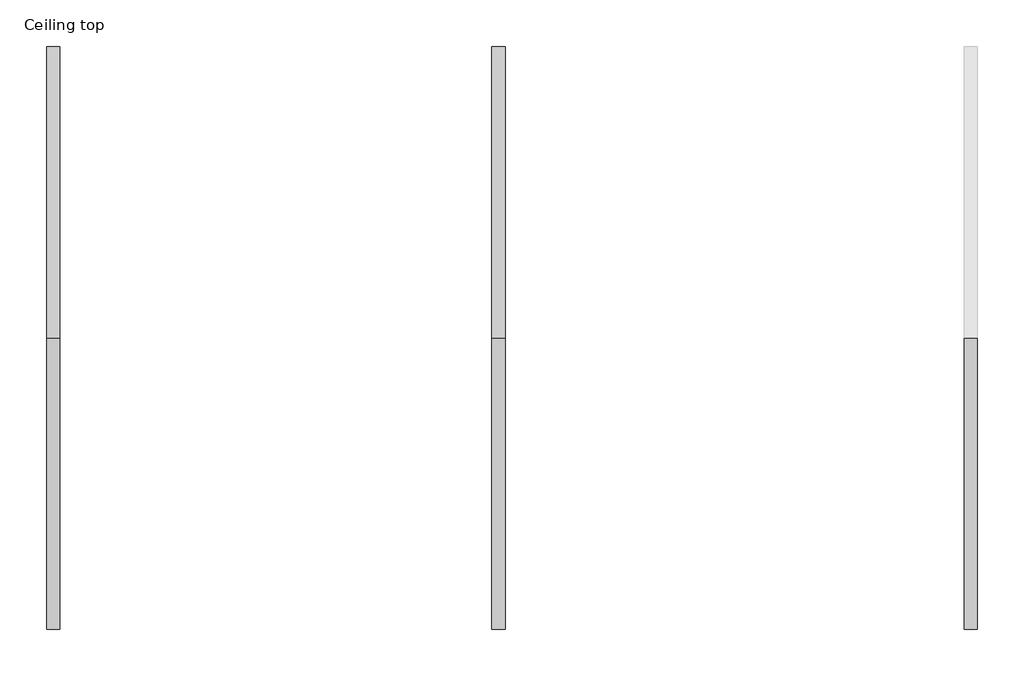
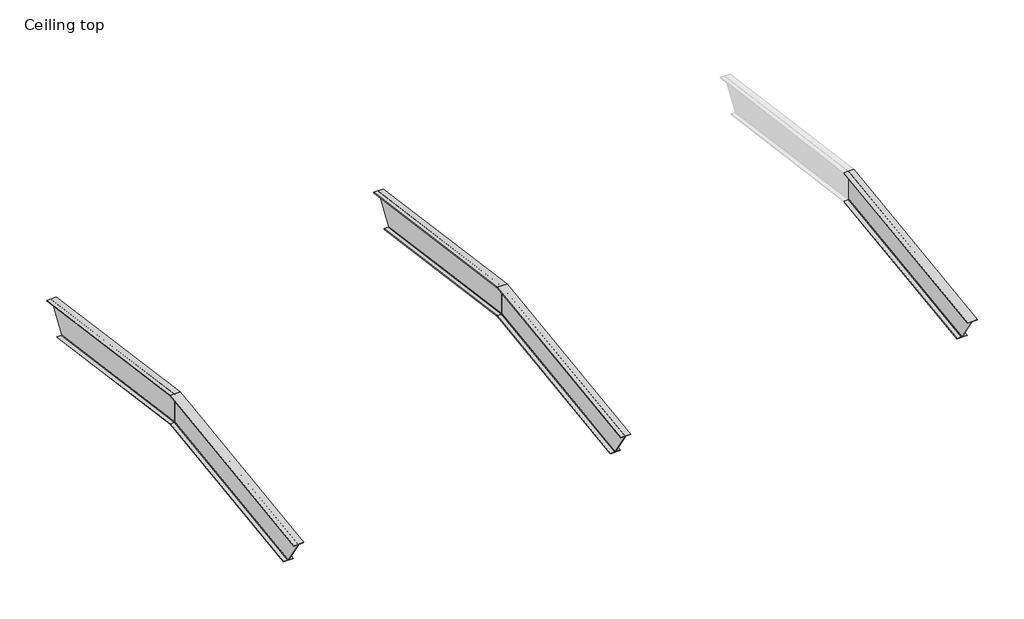
# One storey, part 1 of 2: 5 beams.
"""IFC4 building model written with IfcOpenShell, lengths in millimetres."""

from ifc_helpers import new_model, si_unit, frame, origin, place, context, project, spatial, polyline, ellipse_curve, element, save
from ifc_brep_helpers import plane_surface, revolved_surface, advanced_brep

model = new_model("IFC4")

# Units and contexts
model_context = context("Model", 3, world=origin())
ifc_project = project(units=[si_unit("LENGTHUNIT", "METRE", prefix="MILLI")], contexts=[model_context])

# Site, building, storey
site = spatial("IfcSite", under=ifc_project)
building = spatial("IfcBuilding", under=site)
storey = spatial("IfcBuildingStorey", under=building, Name="Ceiling top", Elevation=4718.05)

# Beams
placement = place(None, origin())
element("IfcBeam", 1, ObjectType="W Shapes : W 6X18.5", at=placement, inside=storey, context=model_context, shape_type="AdvancedBrep", body=[
    advanced_brep(
    [(17988.1780052, 4087.4629396, 4314.3781499), (18053.8370052, 4087.4629396, 4314.3781499), (18053.8370052, 7113.2615366, 4727.7884676), (17988.1780052, 7113.2615366, 4727.7884676), (17980.5580052, 4082.8387117, 4321.4371423), (17980.5580052, 7113.2615366, 4735.4792613), (17980.5580052, 3818.6411587, 4724.7409096), (17980.5580052, 7113.2615366, 5174.8799434), (17988.1780052, 3814.0169308, 4731.799902), (17988.1780052, 7113.2615366, 5182.5707371), (18053.8370052, 3814.0169308, 4731.799902), (18053.8370052, 7113.2615366, 5182.5707371), (18053.8370052, 3808.1595755, 4740.7412924), (18053.8370052, 7113.2615366, 5192.3124092), (17901.4370052, 3808.1595755, 4740.7412924), (17901.4370052, 7113.2615366, 5192.3124092), (17901.4370052, 3814.0169308, 4731.799902), (17901.4370052, 7113.2615366, 5182.5707371), (17967.0960052, 3814.0169308, 4731.799902), (17967.0960052, 7113.2615366, 5182.5707371), (17974.7160052, 3818.6411587, 4724.7409096), (17974.7160052, 7113.2615366, 5174.8799434), (17974.7160052, 4082.8387117, 4321.4371423), (17974.7160052, 7113.2615366, 4735.4792613), (17967.0960052, 4087.4629396, 4314.3781499), (17967.0960052, 7113.2615366, 4727.7884676), (17901.4370052, 4087.4629396, 4314.3781499), (17901.4370052, 7113.2615366, 4727.7884676), (17901.4370052, 4093.3202949, 4305.4367595), (17901.4370052, 7113.2615366, 4718.0467955), (18053.8370052, 4093.3202949, 4305.4367595), (18053.8370052, 7113.2615366, 4718.0467955)],
    [
        (0, 1),
        (1, 2),
        (2, 3),
        (3, 0),
        (4, 0, ellipse_curve(frame((17988.1780052, 4082.8387117, 4321.4371423), z_axis=(0.0, -0.8364953080573767, -0.5479740866117618), x_axis=(0.0, 0.5479740866117613, -0.8364953080573769)), 8.4387711, 7.62)),
        (3, 5, ellipse_curve(frame((17988.1780052, 7113.2615366, 4735.4792613), z_axis=(0.0, 1.0, 0.0), x_axis=(0.0, 0.0, 1.0)), 7.6907937, 7.62)),
        (5, 4),
        (6, 4),
        (5, 7),
        (7, 6),
        (8, 6, ellipse_curve(frame((17988.1780052, 3818.6411587, 4724.7409096), z_axis=(0.0, -0.8364953080573767, -0.5479740866117618), x_axis=(0.0, 0.5479740866117613, -0.8364953080573769)), 8.4387711, 7.62)),
        (7, 9, ellipse_curve(frame((17988.1780052, 7113.2615366, 5174.8799434), z_axis=(0.0, 1.0, 0.0), x_axis=(0.0, 0.0, 1.0)), 7.6907937, 7.62)),
        (9, 8),
        (10, 8),
        (9, 11),
        (11, 10),
        (12, 10),
        (11, 13),
        (13, 12),
        (14, 12),
        (13, 15),
        (15, 14),
        (16, 14),
        (15, 17),
        (17, 16),
        (18, 16),
        (17, 19),
        (19, 18),
        (20, 18, ellipse_curve(frame((17967.0960052, 3818.6411587, 4724.7409096), z_axis=(0.0, -0.8364953080573767, -0.5479740866117618), x_axis=(0.0, 0.5479740866117613, -0.8364953080573769)), 8.4387711, 7.62)),
        (19, 21, ellipse_curve(frame((17967.0960052, 7113.2615366, 5174.8799434), z_axis=(0.0, 1.0, 0.0), x_axis=(0.0, 0.0, 1.0)), 7.6907937, 7.62)),
        (21, 20),
        (22, 20),
        (21, 23),
        (23, 22),
        (24, 22, ellipse_curve(frame((17967.0960052, 4082.8387117, 4321.4371423), z_axis=(0.0, -0.8364953080573767, -0.5479740866117618), x_axis=(0.0, 0.5479740866117613, -0.8364953080573769)), 8.4387711, 7.62)),
        (23, 25, ellipse_curve(frame((17967.0960052, 7113.2615366, 4735.4792613), z_axis=(0.0, 1.0, 0.0), x_axis=(0.0, 0.0, 1.0)), 7.6907937, 7.62)),
        (25, 24),
        (26, 24),
        (25, 27),
        (27, 26),
        (28, 26),
        (27, 29),
        (29, 28),
        (30, 28),
        (29, 31),
        (31, 30),
        (1, 30),
        (31, 2),
    ],
    [
        plane_surface(frame((18053.8370052, 3870.4622337, 4284.7296694), z_axis=(0.0, -0.13537083308413533, 0.9907950027882192), x_axis=(0.0, 0.9907950027882192, 0.13537083308413533))),
        revolved_surface(polyline([(17980.5580052, 7114.293062347846, 4735.620197080616), (17980.5580052, 4079.246009561649, 4320.946276815561)]), (17988.1780052, 3869.430708, 4292.2795273), (0.0, 0.9907950027882191, 0.1353708330841353)),
        plane_surface(frame((17980.5580052, 3869.430708, 4292.2795273), z_axis=(1.0, 0.0, 0.0), x_axis=(0.0, 0.9907950027882192, 0.13537083308413533))),
        revolved_surface(polyline([(17980.5580052, 7114.293062345409, 5175.020879198452), (17980.5580052, 3815.0484565475394, 4724.2500440828635)]), (17988.1780052, 3810.4962036, 4723.6280766), (0.0, 0.9907950027882191, 0.1353708330841353)),
        plane_surface(frame((17988.1780052, 3809.4646778, 4731.1779345), z_axis=(0.0, 0.13537083308413533, -0.9907950027882192), x_axis=(0.0, 0.9907950027882192, 0.13537083308413533))),
        plane_surface(frame((18053.8370052, 3809.4646778, 4731.1779345), z_axis=(1.0, 0.0, 0.0), x_axis=(0.0, 0.9907950027882192, 0.13537083308413533))),
        plane_surface(frame((18053.8370052, 3808.1580786, 4740.7410879), z_axis=(0.0, -0.13537083308413533, 0.9907950027882192), x_axis=(0.0, 0.9907950027882192, 0.13537083308413533))),
        plane_surface(frame((17901.4370052, 3808.1580786, 4740.7410879), z_axis=(-1.0, 0.0, 0.0), x_axis=(0.0, 0.9907950027882192, 0.13537083308413533))),
        plane_surface(frame((17901.4370052, 3809.4646778, 4731.1779345), z_axis=(0.0, 0.13537083308413533, -0.9907950027882192), x_axis=(0.0, 0.9907950027882192, 0.13537083308413533))),
        revolved_surface(polyline([(17959.476005200002, 7114.293062345409, 5175.020879198452), (17959.476005200002, 3815.0484565475394, 4724.2500440828635)]), (17967.0960052, 3810.4962036, 4723.6280766), (0.0, 0.9907950027882191, 0.1353708330841353)),
        plane_surface(frame((17974.7160052, 3810.4962036, 4723.6280766), z_axis=(-1.0, 0.0, 0.0), x_axis=(0.0, 0.9907950027882192, 0.13537083308413533))),
        revolved_surface(polyline([(17959.476005200002, 7114.293062347846, 4735.620197080616), (17959.476005200002, 4079.246009561649, 4320.946276815561)]), (17967.0960052, 3869.430708, 4292.2795273), (0.0, 0.9907950027882191, 0.1353708330841353)),
        plane_surface(frame((17967.0960052, 3870.4622337, 4284.7296694), z_axis=(0.0, -0.13537083308413533, 0.9907950027882192), x_axis=(0.0, 0.9907950027882192, 0.13537083308413533))),
        plane_surface(frame((17901.4370052, 3870.4622337, 4284.7296694), z_axis=(-1.0, 0.0, 0.0), x_axis=(0.0, 0.9907950027882192, 0.13537083308413533))),
        plane_surface(frame((17901.4370052, 3871.768833, 4275.166516), z_axis=(0.0, 0.13537083308413533, -0.9907950027882192), x_axis=(0.0, 0.9907950027882192, 0.13537083308413533))),
        plane_surface(frame((18053.8370052, 3871.768833, 4275.166516), z_axis=(1.0, 0.0, 0.0), x_axis=(0.0, 0.9907950027882192, 0.13537083308413533))),
        plane_surface(frame((17977.6405771, 7113.2615366, 5192.3156137), z_axis=(0.0, 1.0, 0.0), x_axis=(0.0, 0.0, -1.0))),
        plane_surface(frame((17977.6405771, 4093.3183681, 4305.4397008), z_axis=(0.0, -0.8364953080573767, -0.5479740866117618), x_axis=(1.0, 0.0, 0.0))),
    ],
    [
        (0, [[1, 2, 3, 4]]),
        (1, [[5, -4, 6, 7]]),
        (2, [[8, -7, 9, 10]]),
        (3, [[11, -10, 12, 13]]),
        (4, [[14, -13, 15, 16]]),
        (5, [[17, -16, 18, 19]]),
        (6, [[20, -19, 21, 22]]),
        (7, [[23, -22, 24, 25]]),
        (8, [[26, -25, 27, 28]]),
        (9, [[29, -28, 30, 31]]),
        (10, [[32, -31, 33, 34]]),
        (11, [[35, -34, 36, 37]]),
        (12, [[38, -37, 39, 40]]),
        (13, [[41, -40, 42, 43]]),
        (14, [[44, -43, 45, 46]]),
        (15, [[47, -46, 48, -2]]),
        (16, [[-48, -45, -42, -39, -36, -33, -30, -27, -24, -21, -18, -15, -12, -9, -6, -3]]),
        (17, [[-1, -5, -8, -11, -14, -17, -20, -23, -26, -29, -32, -35, -38, -41, -44, -47]]),
    ],
),
])
element("IfcBeam", 2, ObjectType="W Shapes : W 6X18.5", at=placement, inside=storey, context=model_context, shape_type="AdvancedBrep", body=[
    advanced_brep(
    [(12635.1280052, 7113.2615366, 4727.7884676), (12700.7870052, 7113.2615366, 4727.7884676), (12700.7870052, 10139.0601337, 4314.3781499), (12635.1280052, 10139.0601337, 4314.3781499), (12627.5080052, 7113.2615366, 4735.4792613), (12627.5080052, 10143.6843616, 4321.4371423), (12627.5080052, 7113.2615366, 5174.8799434), (12627.5080052, 10407.8819145, 4724.7409096), (12635.1280052, 7113.2615366, 5182.5707371), (12635.1280052, 10412.5061424, 4731.799902), (12700.7870052, 7113.2615366, 5182.5707371), (12700.7870052, 10412.5061424, 4731.799902), (12700.7870052, 7113.2615366, 5192.3124092), (12700.7870052, 10418.3634977, 4740.7412924), (12548.3870052, 7113.2615366, 5192.3124092), (12548.3870052, 10418.3634977, 4740.7412924), (12548.3870052, 7113.2615366, 5182.5707371), (12548.3870052, 10412.5061424, 4731.799902), (12614.0460052, 7113.2615366, 5182.5707371), (12614.0460052, 10412.5061424, 4731.799902), (12621.6660052, 7113.2615366, 5174.8799434), (12621.6660052, 10407.8819145, 4724.7409096), (12621.6660052, 7113.2615366, 4735.4792613), (12621.6660052, 10143.6843616, 4321.4371423), (12614.0460052, 7113.2615366, 4727.7884676), (12614.0460052, 10139.0601337, 4314.3781499), (12548.3870052, 7113.2615366, 4727.7884676), (12548.3870052, 10139.0601337, 4314.3781499), (12548.3870052, 7113.2615366, 4718.0467955), (12548.3870052, 10133.2027784, 4305.4367595), (12700.7870052, 7113.2615366, 4718.0467955), (12700.7870052, 10133.2027784, 4305.4367595)],
    [
        (0, 1),
        (1, 2),
        (2, 3),
        (3, 0),
        (4, 0, ellipse_curve(frame((12635.1280052, 7113.2615366, 4735.4792613), z_axis=(0.0, -1.0, 0.0), x_axis=(0.0, 0.0, -1.0)), 7.6907937, 7.62)),
        (3, 5, ellipse_curve(frame((12635.1280052, 10143.6843616, 4321.4371423), z_axis=(0.0, 0.836495308057375, -0.5479740866117643), x_axis=(0.0, 0.547974086611764, 0.8364953080573752)), 8.4387711, 7.62)),
        (5, 4),
        (6, 4),
        (5, 7),
        (7, 6),
        (8, 6, ellipse_curve(frame((12635.1280052, 7113.2615366, 5174.8799434), z_axis=(0.0, -1.0, 0.0), x_axis=(0.0, 0.0, -1.0)), 7.6907937, 7.62)),
        (7, 9, ellipse_curve(frame((12635.1280052, 10407.8819145, 4724.7409096), z_axis=(0.0, 0.836495308057375, -0.5479740866117643), x_axis=(0.0, 0.547974086611764, 0.8364953080573752)), 8.4387711, 7.62)),
        (9, 8),
        (10, 8),
        (9, 11),
        (11, 10),
        (12, 10),
        (11, 13),
        (13, 12),
        (14, 12),
        (13, 15),
        (15, 14),
        (16, 14),
        (15, 17),
        (17, 16),
        (18, 16),
        (17, 19),
        (19, 18),
        (20, 18, ellipse_curve(frame((12614.0460052, 7113.2615366, 5174.8799434), z_axis=(0.0, -1.0, 0.0), x_axis=(0.0, 0.0, -1.0)), 7.6907937, 7.62)),
        (19, 21, ellipse_curve(frame((12614.0460052, 10407.8819145, 4724.7409096), z_axis=(0.0, 0.836495308057375, -0.5479740866117643), x_axis=(0.0, 0.547974086611764, 0.8364953080573752)), 8.4387711, 7.62)),
        (21, 20),
        (22, 20),
        (21, 23),
        (23, 22),
        (24, 22, ellipse_curve(frame((12614.0460052, 7113.2615366, 4735.4792613), z_axis=(0.0, -1.0, 0.0), x_axis=(0.0, 0.0, -1.0)), 7.6907937, 7.62)),
        (23, 25, ellipse_curve(frame((12614.0460052, 10143.6843616, 4321.4371423), z_axis=(0.0, 0.836495308057375, -0.5479740866117643), x_axis=(0.0, 0.547974086611764, 0.8364953080573752)), 8.4387711, 7.62)),
        (25, 24),
        (26, 24),
        (25, 27),
        (27, 26),
        (28, 26),
        (27, 29),
        (29, 28),
        (30, 28),
        (29, 31),
        (31, 30),
        (1, 30),
        (31, 2),
    ],
    [
        plane_surface(frame((12700.7870052, 7050.9569516, 4736.3010494), z_axis=(0.0, 0.1353708330841357, 0.9907950027882191), x_axis=(0.0, 0.9907950027882191, -0.1353708330841357))),
        revolved_surface(polyline([(12627.5080052, 10147.277063747912, 4320.946276885532), (12627.5080052, 7112.230010863546, 4735.620197164001)]), (12635.1280052, 7051.9884774, 4743.8509074), (0.0, 0.9907950027882191, -0.1353708330841357)),
        plane_surface(frame((12627.5080052, 7051.9884774, 4743.8509074), z_axis=(1.0, 0.0, 0.0), x_axis=(0.0, 0.9907950027882191, -0.1353708330841357))),
        revolved_surface(polyline([(12627.5080052, 10411.474616650441, 4724.25004406808), (12627.5080052, 7112.230010852571, 5175.020879183669)]), (12635.1280052, 7110.9229818, 5175.1994566), (0.0, 0.9907950027882191, -0.1353708330841357)),
        plane_surface(frame((12635.1280052, 7111.9545075, 5182.7493145), z_axis=(0.0, -0.1353708330841357, -0.9907950027882191), x_axis=(0.0, 0.9907950027882191, -0.1353708330841357))),
        plane_surface(frame((12700.7870052, 7111.9545075, 5182.7493145), z_axis=(1.0, 0.0, 0.0), x_axis=(0.0, 0.9907950027882191, -0.1353708330841357))),
        plane_surface(frame((12700.7870052, 7113.2611068, 5192.3124679), z_axis=(0.0, 0.1353708330841357, 0.9907950027882191), x_axis=(0.0, 0.9907950027882191, -0.1353708330841357))),
        plane_surface(frame((12548.3870052, 7113.2611068, 5192.3124679), z_axis=(-1.0, 0.0, 0.0), x_axis=(0.0, 0.9907950027882191, -0.1353708330841357))),
        plane_surface(frame((12548.3870052, 7111.9545075, 5182.7493145), z_axis=(0.0, -0.1353708330841357, -0.9907950027882191), x_axis=(0.0, 0.9907950027882191, -0.1353708330841357))),
        revolved_surface(polyline([(12606.426005199999, 10411.474616650441, 4724.25004406808), (12606.426005199999, 7112.230010852571, 5175.020879183669)]), (12614.0460052, 7110.9229818, 5175.1994566), (0.0, 0.9907950027882191, -0.1353708330841357)),
        plane_surface(frame((12621.6660052, 7110.9229818, 5175.1994566), z_axis=(-1.0, 0.0, 0.0), x_axis=(0.0, 0.9907950027882191, -0.1353708330841357))),
        revolved_surface(polyline([(12606.426005199999, 10147.277063747912, 4320.946276885532), (12606.426005199999, 7112.230010863546, 4735.620197164001)]), (12614.0460052, 7051.9884774, 4743.8509074), (0.0, 0.9907950027882191, -0.1353708330841357)),
        plane_surface(frame((12614.0460052, 7050.9569516, 4736.3010494), z_axis=(0.0, 0.1353708330841357, 0.9907950027882191), x_axis=(0.0, 0.9907950027882191, -0.1353708330841357))),
        plane_surface(frame((12548.3870052, 7050.9569516, 4736.3010494), z_axis=(-1.0, 0.0, 0.0), x_axis=(0.0, 0.9907950027882191, -0.1353708330841357))),
        plane_surface(frame((12548.3870052, 7049.6503524, 4726.7378961), z_axis=(0.0, -0.1353708330841357, -0.9907950027882191), x_axis=(0.0, 0.9907950027882191, -0.1353708330841357))),
        plane_surface(frame((12700.7870052, 7049.6503524, 4726.7378961), z_axis=(1.0, 0.0, 0.0), x_axis=(0.0, 0.9907950027882191, -0.1353708330841357))),
        plane_surface(frame((12624.5905771, 7113.2615366, 5192.3156137), z_axis=(0.0, -1.0, 0.0), x_axis=(0.0, 0.0, 1.0))),
        plane_surface(frame((12624.5905771, 10418.3654245, 4740.7442336), z_axis=(0.0, 0.836495308057375, -0.5479740866117643), x_axis=(1.0, 0.0, 0.0))),
    ],
    [
        (0, [[1, 2, 3, 4]]),
        (1, [[5, -4, 6, 7]]),
        (2, [[8, -7, 9, 10]]),
        (3, [[11, -10, 12, 13]]),
        (4, [[14, -13, 15, 16]]),
        (5, [[17, -16, 18, 19]]),
        (6, [[20, -19, 21, 22]]),
        (7, [[23, -22, 24, 25]]),
        (8, [[26, -25, 27, 28]]),
        (9, [[29, -28, 30, 31]]),
        (10, [[32, -31, 33, 34]]),
        (11, [[35, -34, 36, 37]]),
        (12, [[38, -37, 39, 40]]),
        (13, [[41, -40, 42, 43]]),
        (14, [[44, -43, 45, 46]]),
        (15, [[47, -46, 48, -2]]),
        (16, [[-1, -5, -8, -11, -14, -17, -20, -23, -26, -29, -32, -35, -38, -41, -44, -47]]),
        (17, [[-48, -45, -42, -39, -36, -33, -30, -27, -24, -21, -18, -15, -12, -9, -6, -3]]),
    ],
),
])
element("IfcBeam", 3, ObjectType="W Shapes : W 6X18.5", at=placement, inside=storey, context=model_context, shape_type="AdvancedBrep", body=[
    advanced_brep(
    [(12635.1280052, 4087.4629396, 4314.3781499), (12700.7870052, 4087.4629396, 4314.3781499), (12700.7870052, 7113.2615366, 4727.7884676), (12635.1280052, 7113.2615366, 4727.7884676), (12627.5080052, 4082.8387117, 4321.4371423), (12627.5080052, 7113.2615366, 4735.4792613), (12627.5080052, 3818.6411587, 4724.7409096), (12627.5080052, 7113.2615366, 5174.8799434), (12635.1280052, 3814.0169308, 4731.799902), (12635.1280052, 7113.2615366, 5182.5707371), (12700.7870052, 3814.0169308, 4731.799902), (12700.7870052, 7113.2615366, 5182.5707371), (12700.7870052, 3808.1595755, 4740.7412924), (12700.7870052, 7113.2615366, 5192.3124092), (12548.3870052, 3808.1595755, 4740.7412924), (12548.3870052, 7113.2615366, 5192.3124092), (12548.3870052, 3814.0169308, 4731.799902), (12548.3870052, 7113.2615366, 5182.5707371), (12614.0460052, 3814.0169308, 4731.799902), (12614.0460052, 7113.2615366, 5182.5707371), (12621.6660052, 3818.6411587, 4724.7409096), (12621.6660052, 7113.2615366, 5174.8799434), (12621.6660052, 4082.8387117, 4321.4371423), (12621.6660052, 7113.2615366, 4735.4792613), (12614.0460052, 4087.4629396, 4314.3781499), (12614.0460052, 7113.2615366, 4727.7884676), (12548.3870052, 4087.4629396, 4314.3781499), (12548.3870052, 7113.2615366, 4727.7884676), (12548.3870052, 4093.3202949, 4305.4367595), (12548.3870052, 7113.2615366, 4718.0467955), (12700.7870052, 4093.3202949, 4305.4367595), (12700.7870052, 7113.2615366, 4718.0467955)],
    [
        (0, 1),
        (1, 2),
        (2, 3),
        (3, 0),
        (4, 0, ellipse_curve(frame((12635.1280052, 4082.8387117, 4321.4371423), z_axis=(0.0, -0.8364953080573767, -0.5479740866117618), x_axis=(0.0, 0.5479740866117613, -0.8364953080573769)), 8.4387711, 7.62)),
        (3, 5, ellipse_curve(frame((12635.1280052, 7113.2615366, 4735.4792613), z_axis=(0.0, 1.0, 0.0), x_axis=(0.0, 0.0, 1.0)), 7.6907937, 7.62)),
        (5, 4),
        (6, 4),
        (5, 7),
        (7, 6),
        (8, 6, ellipse_curve(frame((12635.1280052, 3818.6411587, 4724.7409096), z_axis=(0.0, -0.8364953080573767, -0.5479740866117618), x_axis=(0.0, 0.5479740866117613, -0.8364953080573769)), 8.4387711, 7.62)),
        (7, 9, ellipse_curve(frame((12635.1280052, 7113.2615366, 5174.8799434), z_axis=(0.0, 1.0, 0.0), x_axis=(0.0, 0.0, 1.0)), 7.6907937, 7.62)),
        (9, 8),
        (10, 8),
        (9, 11),
        (11, 10),
        (12, 10),
        (11, 13),
        (13, 12),
        (14, 12),
        (13, 15),
        (15, 14),
        (16, 14),
        (15, 17),
        (17, 16),
        (18, 16),
        (17, 19),
        (19, 18),
        (20, 18, ellipse_curve(frame((12614.0460052, 3818.6411587, 4724.7409096), z_axis=(0.0, -0.8364953080573767, -0.5479740866117618), x_axis=(0.0, 0.5479740866117613, -0.8364953080573769)), 8.4387711, 7.62)),
        (19, 21, ellipse_curve(frame((12614.0460052, 7113.2615366, 5174.8799434), z_axis=(0.0, 1.0, 0.0), x_axis=(0.0, 0.0, 1.0)), 7.6907937, 7.62)),
        (21, 20),
        (22, 20),
        (21, 23),
        (23, 22),
        (24, 22, ellipse_curve(frame((12614.0460052, 4082.8387117, 4321.4371423), z_axis=(0.0, -0.8364953080573767, -0.5479740866117618), x_axis=(0.0, 0.5479740866117613, -0.8364953080573769)), 8.4387711, 7.62)),
        (23, 25, ellipse_curve(frame((12614.0460052, 7113.2615366, 4735.4792613), z_axis=(0.0, 1.0, 0.0), x_axis=(0.0, 0.0, 1.0)), 7.6907937, 7.62)),
        (25, 24),
        (26, 24),
        (25, 27),
        (27, 26),
        (28, 26),
        (27, 29),
        (29, 28),
        (30, 28),
        (29, 31),
        (31, 30),
        (1, 30),
        (31, 2),
    ],
    [
        plane_surface(frame((12700.7870052, 3870.4622337, 4284.7296694), z_axis=(0.0, -0.13537083308413533, 0.9907950027882192), x_axis=(0.0, 0.9907950027882192, 0.13537083308413533))),
        revolved_surface(polyline([(12627.5080052, 7114.293062347846, 4735.620197080616), (12627.5080052, 4079.246009561649, 4320.946276815561)]), (12635.1280052, 3869.430708, 4292.2795273), (0.0, 0.9907950027882191, 0.1353708330841353)),
        plane_surface(frame((12627.5080052, 3869.430708, 4292.2795273), z_axis=(1.0, 0.0, 0.0), x_axis=(0.0, 0.9907950027882192, 0.13537083308413533))),
        revolved_surface(polyline([(12627.5080052, 7114.293062345409, 5175.020879198452), (12627.5080052, 3815.0484565475394, 4724.2500440828635)]), (12635.1280052, 3810.4962036, 4723.6280766), (0.0, 0.9907950027882191, 0.1353708330841353)),
        plane_surface(frame((12635.1280052, 3809.4646778, 4731.1779345), z_axis=(0.0, 0.13537083308413533, -0.9907950027882192), x_axis=(0.0, 0.9907950027882192, 0.13537083308413533))),
        plane_surface(frame((12700.7870052, 3809.4646778, 4731.1779345), z_axis=(1.0, 0.0, 0.0), x_axis=(0.0, 0.9907950027882192, 0.13537083308413533))),
        plane_surface(frame((12700.7870052, 3808.1580786, 4740.7410879), z_axis=(0.0, -0.13537083308413533, 0.9907950027882192), x_axis=(0.0, 0.9907950027882192, 0.13537083308413533))),
        plane_surface(frame((12548.3870052, 3808.1580786, 4740.7410879), z_axis=(-1.0, 0.0, 0.0), x_axis=(0.0, 0.9907950027882192, 0.13537083308413533))),
        plane_surface(frame((12548.3870052, 3809.4646778, 4731.1779345), z_axis=(0.0, 0.13537083308413533, -0.9907950027882192), x_axis=(0.0, 0.9907950027882192, 0.13537083308413533))),
        revolved_surface(polyline([(12606.426005199999, 7114.293062345409, 5175.020879198452), (12606.426005199999, 3815.0484565475394, 4724.2500440828635)]), (12614.0460052, 3810.4962036, 4723.6280766), (0.0, 0.9907950027882191, 0.1353708330841353)),
        plane_surface(frame((12621.6660052, 3810.4962036, 4723.6280766), z_axis=(-1.0, 0.0, 0.0), x_axis=(0.0, 0.9907950027882192, 0.13537083308413533))),
        revolved_surface(polyline([(12606.426005199999, 7114.293062347846, 4735.620197080616), (12606.426005199999, 4079.246009561649, 4320.946276815561)]), (12614.0460052, 3869.430708, 4292.2795273), (0.0, 0.9907950027882191, 0.1353708330841353)),
        plane_surface(frame((12614.0460052, 3870.4622337, 4284.7296694), z_axis=(0.0, -0.13537083308413533, 0.9907950027882192), x_axis=(0.0, 0.9907950027882192, 0.13537083308413533))),
        plane_surface(frame((12548.3870052, 3870.4622337, 4284.7296694), z_axis=(-1.0, 0.0, 0.0), x_axis=(0.0, 0.9907950027882192, 0.13537083308413533))),
        plane_surface(frame((12548.3870052, 3871.768833, 4275.166516), z_axis=(0.0, 0.13537083308413533, -0.9907950027882192), x_axis=(0.0, 0.9907950027882192, 0.13537083308413533))),
        plane_surface(frame((12700.7870052, 3871.768833, 4275.166516), z_axis=(1.0, 0.0, 0.0), x_axis=(0.0, 0.9907950027882192, 0.13537083308413533))),
        plane_surface(frame((12624.5905771, 7113.2615366, 5192.3156137), z_axis=(0.0, 1.0, 0.0), x_axis=(0.0, 0.0, -1.0))),
        plane_surface(frame((12624.5905771, 4093.3183681, 4305.4397008), z_axis=(0.0, -0.8364953080573767, -0.5479740866117618), x_axis=(1.0, 0.0, 0.0))),
    ],
    [
        (0, [[1, 2, 3, 4]]),
        (1, [[5, -4, 6, 7]]),
        (2, [[8, -7, 9, 10]]),
        (3, [[11, -10, 12, 13]]),
        (4, [[14, -13, 15, 16]]),
        (5, [[17, -16, 18, 19]]),
        (6, [[20, -19, 21, 22]]),
        (7, [[23, -22, 24, 25]]),
        (8, [[26, -25, 27, 28]]),
        (9, [[29, -28, 30, 31]]),
        (10, [[32, -31, 33, 34]]),
        (11, [[35, -34, 36, 37]]),
        (12, [[38, -37, 39, 40]]),
        (13, [[41, -40, 42, 43]]),
        (14, [[44, -43, 45, 46]]),
        (15, [[47, -46, 48, -2]]),
        (16, [[-48, -45, -42, -39, -36, -33, -30, -27, -24, -21, -18, -15, -12, -9, -6, -3]]),
        (17, [[-1, -5, -8, -11, -14, -17, -20, -23, -26, -29, -32, -35, -38, -41, -44, -47]]),
    ],
),
])
element("IfcBeam", 4, ObjectType="W Shapes : W 6X18.5", at=placement, inside=storey, context=model_context, shape_type="AdvancedBrep", body=[
    advanced_brep(
    [(7586.8780052, 7113.2615366, 4727.7884676), (7652.5370052, 7113.2615366, 4727.7884676), (7652.5370052, 10139.0601337, 4314.3781499), (7586.8780052, 10139.0601337, 4314.3781499), (7579.2580052, 7113.2615366, 4735.4792613), (7579.2580052, 10143.6843616, 4321.4371423), (7579.2580052, 7113.2615366, 5174.8799434), (7579.2580052, 10407.8819145, 4724.7409096), (7586.8780052, 7113.2615366, 5182.5707371), (7586.8780052, 10412.5061424, 4731.799902), (7652.5370052, 7113.2615366, 5182.5707371), (7652.5370052, 10412.5061424, 4731.799902), (7652.5370052, 7113.2615366, 5192.3124092), (7652.5370052, 10418.3634977, 4740.7412924), (7500.1370052, 7113.2615366, 5192.3124092), (7500.1370052, 10418.3634977, 4740.7412924), (7500.1370052, 7113.2615366, 5182.5707371), (7500.1370052, 10412.5061424, 4731.799902), (7565.7960052, 7113.2615366, 5182.5707371), (7565.7960052, 10412.5061424, 4731.799902), (7573.4160052, 7113.2615366, 5174.8799434), (7573.4160052, 10407.8819145, 4724.7409096), (7573.4160052, 7113.2615366, 4735.4792613), (7573.4160052, 10143.6843616, 4321.4371423), (7565.7960052, 7113.2615366, 4727.7884676), (7565.7960052, 10139.0601337, 4314.3781499), (7500.1370052, 7113.2615366, 4727.7884676), (7500.1370052, 10139.0601337, 4314.3781499), (7500.1370052, 7113.2615366, 4718.0467955), (7500.1370052, 10133.2027784, 4305.4367595), (7652.5370052, 7113.2615366, 4718.0467955), (7652.5370052, 10133.2027784, 4305.4367595)],
    [
        (0, 1),
        (1, 2),
        (2, 3),
        (3, 0),
        (4, 0, ellipse_curve(frame((7586.8780052, 7113.2615366, 4735.4792613), z_axis=(0.0, -1.0, 0.0), x_axis=(0.0, 0.0, -1.0)), 7.6907937, 7.62)),
        (3, 5, ellipse_curve(frame((7586.8780052, 10143.6843616, 4321.4371423), z_axis=(0.0, 0.836495308057375, -0.5479740866117643), x_axis=(0.0, 0.547974086611764, 0.8364953080573752)), 8.4387711, 7.62)),
        (5, 4),
        (6, 4),
        (5, 7),
        (7, 6),
        (8, 6, ellipse_curve(frame((7586.8780052, 7113.2615366, 5174.8799434), z_axis=(0.0, -1.0, 0.0), x_axis=(0.0, 0.0, -1.0)), 7.6907937, 7.62)),
        (7, 9, ellipse_curve(frame((7586.8780052, 10407.8819145, 4724.7409096), z_axis=(0.0, 0.836495308057375, -0.5479740866117643), x_axis=(0.0, 0.547974086611764, 0.8364953080573752)), 8.4387711, 7.62)),
        (9, 8),
        (10, 8),
        (9, 11),
        (11, 10),
        (12, 10),
        (11, 13),
        (13, 12),
        (14, 12),
        (13, 15),
        (15, 14),
        (16, 14),
        (15, 17),
        (17, 16),
        (18, 16),
        (17, 19),
        (19, 18),
        (20, 18, ellipse_curve(frame((7565.7960052, 7113.2615366, 5174.8799434), z_axis=(0.0, -1.0, 0.0), x_axis=(0.0, 0.0, -1.0)), 7.6907937, 7.62)),
        (19, 21, ellipse_curve(frame((7565.7960052, 10407.8819145, 4724.7409096), z_axis=(0.0, 0.836495308057375, -0.5479740866117643), x_axis=(0.0, 0.547974086611764, 0.8364953080573752)), 8.4387711, 7.62)),
        (21, 20),
        (22, 20),
        (21, 23),
        (23, 22),
        (24, 22, ellipse_curve(frame((7565.7960052, 7113.2615366, 4735.4792613), z_axis=(0.0, -1.0, 0.0), x_axis=(0.0, 0.0, -1.0)), 7.6907937, 7.62)),
        (23, 25, ellipse_curve(frame((7565.7960052, 10143.6843616, 4321.4371423), z_axis=(0.0, 0.836495308057375, -0.5479740866117643), x_axis=(0.0, 0.547974086611764, 0.8364953080573752)), 8.4387711, 7.62)),
        (25, 24),
        (26, 24),
        (25, 27),
        (27, 26),
        (28, 26),
        (27, 29),
        (29, 28),
        (30, 28),
        (29, 31),
        (31, 30),
        (1, 30),
        (31, 2),
    ],
    [
        plane_surface(frame((7652.5370052, 7050.9569516, 4736.3010494), z_axis=(0.0, 0.1353708330841357, 0.9907950027882191), x_axis=(0.0, 0.9907950027882191, -0.1353708330841357))),
        revolved_surface(polyline([(7579.2580052, 10147.277063747912, 4320.946276885532), (7579.2580052, 7112.230010863546, 4735.620197164001)]), (7586.8780052, 7051.9884774, 4743.8509074), (0.0, 0.9907950027882191, -0.1353708330841357)),
        plane_surface(frame((7579.2580052, 7051.9884774, 4743.8509074), z_axis=(1.0, 0.0, 0.0), x_axis=(0.0, 0.9907950027882191, -0.1353708330841357))),
        revolved_surface(polyline([(7579.2580052, 10411.474616650441, 4724.25004406808), (7579.2580052, 7112.230010852571, 5175.020879183669)]), (7586.8780052, 7110.9229818, 5175.1994566), (0.0, 0.9907950027882191, -0.1353708330841357)),
        plane_surface(frame((7586.8780052, 7111.9545075, 5182.7493145), z_axis=(0.0, -0.1353708330841357, -0.9907950027882191), x_axis=(0.0, 0.9907950027882191, -0.1353708330841357))),
        plane_surface(frame((7652.5370052, 7111.9545075, 5182.7493145), z_axis=(1.0, 0.0, 0.0), x_axis=(0.0, 0.9907950027882191, -0.1353708330841357))),
        plane_surface(frame((7652.5370052, 7113.2611068, 5192.3124679), z_axis=(0.0, 0.1353708330841357, 0.9907950027882191), x_axis=(0.0, 0.9907950027882191, -0.1353708330841357))),
        plane_surface(frame((7500.1370052, 7113.2611068, 5192.3124679), z_axis=(-1.0, 0.0, 0.0), x_axis=(0.0, 0.9907950027882191, -0.1353708330841357))),
        plane_surface(frame((7500.1370052, 7111.9545075, 5182.7493145), z_axis=(0.0, -0.1353708330841357, -0.9907950027882191), x_axis=(0.0, 0.9907950027882191, -0.1353708330841357))),
        revolved_surface(polyline([(7558.1760052, 10411.474616650441, 4724.25004406808), (7558.1760052, 7112.230010852571, 5175.020879183669)]), (7565.7960052, 7110.9229818, 5175.1994566), (0.0, 0.9907950027882191, -0.1353708330841357)),
        plane_surface(frame((7573.4160052, 7110.9229818, 5175.1994566), z_axis=(-1.0, 0.0, 0.0), x_axis=(0.0, 0.9907950027882191, -0.1353708330841357))),
        revolved_surface(polyline([(7558.1760052, 10147.277063747912, 4320.946276885532), (7558.1760052, 7112.230010863546, 4735.620197164001)]), (7565.7960052, 7051.9884774, 4743.8509074), (0.0, 0.9907950027882191, -0.1353708330841357)),
        plane_surface(frame((7565.7960052, 7050.9569516, 4736.3010494), z_axis=(0.0, 0.1353708330841357, 0.9907950027882191), x_axis=(0.0, 0.9907950027882191, -0.1353708330841357))),
        plane_surface(frame((7500.1370052, 7050.9569516, 4736.3010494), z_axis=(-1.0, 0.0, 0.0), x_axis=(0.0, 0.9907950027882191, -0.1353708330841357))),
        plane_surface(frame((7500.1370052, 7049.6503524, 4726.7378961), z_axis=(0.0, -0.1353708330841357, -0.9907950027882191), x_axis=(0.0, 0.9907950027882191, -0.1353708330841357))),
        plane_surface(frame((7652.5370052, 7049.6503524, 4726.7378961), z_axis=(1.0, 0.0, 0.0), x_axis=(0.0, 0.9907950027882191, -0.1353708330841357))),
        plane_surface(frame((7576.3405771, 7113.2615366, 5192.3156137), z_axis=(0.0, -1.0, 0.0), x_axis=(0.0, 0.0, 1.0))),
        plane_surface(frame((7576.3405771, 10418.3654245, 4740.7442336), z_axis=(0.0, 0.836495308057375, -0.5479740866117643), x_axis=(1.0, 0.0, 0.0))),
    ],
    [
        (0, [[1, 2, 3, 4]]),
        (1, [[5, -4, 6, 7]]),
        (2, [[8, -7, 9, 10]]),
        (3, [[11, -10, 12, 13]]),
        (4, [[14, -13, 15, 16]]),
        (5, [[17, -16, 18, 19]]),
        (6, [[20, -19, 21, 22]]),
        (7, [[23, -22, 24, 25]]),
        (8, [[26, -25, 27, 28]]),
        (9, [[29, -28, 30, 31]]),
        (10, [[32, -31, 33, 34]]),
        (11, [[35, -34, 36, 37]]),
        (12, [[38, -37, 39, 40]]),
        (13, [[41, -40, 42, 43]]),
        (14, [[44, -43, 45, 46]]),
        (15, [[47, -46, 48, -2]]),
        (16, [[-1, -5, -8, -11, -14, -17, -20, -23, -26, -29, -32, -35, -38, -41, -44, -47]]),
        (17, [[-48, -45, -42, -39, -36, -33, -30, -27, -24, -21, -18, -15, -12, -9, -6, -3]]),
    ],
),
])
element("IfcBeam", 5, ObjectType="W Shapes : W 6X18.5", at=placement, inside=storey, context=model_context, shape_type="AdvancedBrep", body=[
    advanced_brep(
    [(7586.8780052, 4087.4629396, 4314.3781499), (7652.5370052, 4087.4629396, 4314.3781499), (7652.5370052, 7113.2615366, 4727.7884676), (7586.8780052, 7113.2615366, 4727.7884676), (7579.2580052, 4082.8387117, 4321.4371423), (7579.2580052, 7113.2615366, 4735.4792613), (7579.2580052, 3818.6411587, 4724.7409096), (7579.2580052, 7113.2615366, 5174.8799434), (7586.8780052, 3814.0169308, 4731.799902), (7586.8780052, 7113.2615366, 5182.5707371), (7652.5370052, 3814.0169308, 4731.799902), (7652.5370052, 7113.2615366, 5182.5707371), (7652.5370052, 3808.1595755, 4740.7412924), (7652.5370052, 7113.2615366, 5192.3124092), (7500.1370052, 3808.1595755, 4740.7412924), (7500.1370052, 7113.2615366, 5192.3124092), (7500.1370052, 3814.0169308, 4731.799902), (7500.1370052, 7113.2615366, 5182.5707371), (7565.7960052, 3814.0169308, 4731.799902), (7565.7960052, 7113.2615366, 5182.5707371), (7573.4160052, 3818.6411587, 4724.7409096), (7573.4160052, 7113.2615366, 5174.8799434), (7573.4160052, 4082.8387117, 4321.4371423), (7573.4160052, 7113.2615366, 4735.4792613), (7565.7960052, 4087.4629396, 4314.3781499), (7565.7960052, 7113.2615366, 4727.7884676), (7500.1370052, 4087.4629396, 4314.3781499), (7500.1370052, 7113.2615366, 4727.7884676), (7500.1370052, 4093.3202949, 4305.4367595), (7500.1370052, 7113.2615366, 4718.0467955), (7652.5370052, 4093.3202949, 4305.4367595), (7652.5370052, 7113.2615366, 4718.0467955)],
    [
        (0, 1),
        (1, 2),
        (2, 3),
        (3, 0),
        (4, 0, ellipse_curve(frame((7586.8780052, 4082.8387117, 4321.4371423), z_axis=(0.0, -0.8364953080573767, -0.5479740866117618), x_axis=(0.0, 0.5479740866117613, -0.8364953080573769)), 8.4387711, 7.62)),
        (3, 5, ellipse_curve(frame((7586.8780052, 7113.2615366, 4735.4792613), z_axis=(0.0, 1.0, 0.0), x_axis=(0.0, 0.0, 1.0)), 7.6907937, 7.62)),
        (5, 4),
        (6, 4),
        (5, 7),
        (7, 6),
        (8, 6, ellipse_curve(frame((7586.8780052, 3818.6411587, 4724.7409096), z_axis=(0.0, -0.8364953080573767, -0.5479740866117618), x_axis=(0.0, 0.5479740866117613, -0.8364953080573769)), 8.4387711, 7.62)),
        (7, 9, ellipse_curve(frame((7586.8780052, 7113.2615366, 5174.8799434), z_axis=(0.0, 1.0, 0.0), x_axis=(0.0, 0.0, 1.0)), 7.6907937, 7.62)),
        (9, 8),
        (10, 8),
        (9, 11),
        (11, 10),
        (12, 10),
        (11, 13),
        (13, 12),
        (14, 12),
        (13, 15),
        (15, 14),
        (16, 14),
        (15, 17),
        (17, 16),
        (18, 16),
        (17, 19),
        (19, 18),
        (20, 18, ellipse_curve(frame((7565.7960052, 3818.6411587, 4724.7409096), z_axis=(0.0, -0.8364953080573767, -0.5479740866117618), x_axis=(0.0, 0.5479740866117613, -0.8364953080573769)), 8.4387711, 7.62)),
        (19, 21, ellipse_curve(frame((7565.7960052, 7113.2615366, 5174.8799434), z_axis=(0.0, 1.0, 0.0), x_axis=(0.0, 0.0, 1.0)), 7.6907937, 7.62)),
        (21, 20),
        (22, 20),
        (21, 23),
        (23, 22),
        (24, 22, ellipse_curve(frame((7565.7960052, 4082.8387117, 4321.4371423), z_axis=(0.0, -0.8364953080573767, -0.5479740866117618), x_axis=(0.0, 0.5479740866117613, -0.8364953080573769)), 8.4387711, 7.62)),
        (23, 25, ellipse_curve(frame((7565.7960052, 7113.2615366, 4735.4792613), z_axis=(0.0, 1.0, 0.0), x_axis=(0.0, 0.0, 1.0)), 7.6907937, 7.62)),
        (25, 24),
        (26, 24),
        (25, 27),
        (27, 26),
        (28, 26),
        (27, 29),
        (29, 28),
        (30, 28),
        (29, 31),
        (31, 30),
        (1, 30),
        (31, 2),
    ],
    [
        plane_surface(frame((7652.5370052, 3870.4622337, 4284.7296694), z_axis=(0.0, -0.13537083308413533, 0.9907950027882192), x_axis=(0.0, 0.9907950027882192, 0.13537083308413533))),
        revolved_surface(polyline([(7579.2580052, 7114.293062347846, 4735.620197080616), (7579.2580052, 4079.246009561649, 4320.946276815561)]), (7586.8780052, 3869.430708, 4292.2795273), (0.0, 0.9907950027882191, 0.1353708330841353)),
        plane_surface(frame((7579.2580052, 3869.430708, 4292.2795273), z_axis=(1.0, 0.0, 0.0), x_axis=(0.0, 0.9907950027882192, 0.13537083308413533))),
        revolved_surface(polyline([(7579.2580052, 7114.293062345409, 5175.020879198452), (7579.2580052, 3815.0484565475394, 4724.2500440828635)]), (7586.8780052, 3810.4962036, 4723.6280766), (0.0, 0.9907950027882191, 0.1353708330841353)),
        plane_surface(frame((7586.8780052, 3809.4646778, 4731.1779345), z_axis=(0.0, 0.13537083308413533, -0.9907950027882192), x_axis=(0.0, 0.9907950027882192, 0.13537083308413533))),
        plane_surface(frame((7652.5370052, 3809.4646778, 4731.1779345), z_axis=(1.0, 0.0, 0.0), x_axis=(0.0, 0.9907950027882192, 0.13537083308413533))),
        plane_surface(frame((7652.5370052, 3808.1580786, 4740.7410879), z_axis=(0.0, -0.13537083308413533, 0.9907950027882192), x_axis=(0.0, 0.9907950027882192, 0.13537083308413533))),
        plane_surface(frame((7500.1370052, 3808.1580786, 4740.7410879), z_axis=(-1.0, 0.0, 0.0), x_axis=(0.0, 0.9907950027882192, 0.13537083308413533))),
        plane_surface(frame((7500.1370052, 3809.4646778, 4731.1779345), z_axis=(0.0, 0.13537083308413533, -0.9907950027882192), x_axis=(0.0, 0.9907950027882192, 0.13537083308413533))),
        revolved_surface(polyline([(7558.1760052, 7114.293062345409, 5175.020879198452), (7558.1760052, 3815.0484565475394, 4724.2500440828635)]), (7565.7960052, 3810.4962036, 4723.6280766), (0.0, 0.9907950027882191, 0.1353708330841353)),
        plane_surface(frame((7573.4160052, 3810.4962036, 4723.6280766), z_axis=(-1.0, 0.0, 0.0), x_axis=(0.0, 0.9907950027882192, 0.13537083308413533))),
        revolved_surface(polyline([(7558.1760052, 7114.293062347846, 4735.620197080616), (7558.1760052, 4079.246009561649, 4320.946276815561)]), (7565.7960052, 3869.430708, 4292.2795273), (0.0, 0.9907950027882191, 0.1353708330841353)),
        plane_surface(frame((7565.7960052, 3870.4622337, 4284.7296694), z_axis=(0.0, -0.13537083308413533, 0.9907950027882192), x_axis=(0.0, 0.9907950027882192, 0.13537083308413533))),
        plane_surface(frame((7500.1370052, 3870.4622337, 4284.7296694), z_axis=(-1.0, 0.0, 0.0), x_axis=(0.0, 0.9907950027882192, 0.13537083308413533))),
        plane_surface(frame((7500.1370052, 3871.768833, 4275.166516), z_axis=(0.0, 0.13537083308413533, -0.9907950027882192), x_axis=(0.0, 0.9907950027882192, 0.13537083308413533))),
        plane_surface(frame((7652.5370052, 3871.768833, 4275.166516), z_axis=(1.0, 0.0, 0.0), x_axis=(0.0, 0.9907950027882192, 0.13537083308413533))),
        plane_surface(frame((7576.3405771, 7113.2615366, 5192.3156137), z_axis=(0.0, 1.0, 0.0), x_axis=(0.0, 0.0, -1.0))),
        plane_surface(frame((7576.3405771, 4093.3183681, 4305.4397008), z_axis=(0.0, -0.8364953080573767, -0.5479740866117618), x_axis=(1.0, 0.0, 0.0))),
    ],
    [
        (0, [[1, 2, 3, 4]]),
        (1, [[5, -4, 6, 7]]),
        (2, [[8, -7, 9, 10]]),
        (3, [[11, -10, 12, 13]]),
        (4, [[14, -13, 15, 16]]),
        (5, [[17, -16, 18, 19]]),
        (6, [[20, -19, 21, 22]]),
        (7, [[23, -22, 24, 25]]),
        (8, [[26, -25, 27, 28]]),
        (9, [[29, -28, 30, 31]]),
        (10, [[32, -31, 33, 34]]),
        (11, [[35, -34, 36, 37]]),
        (12, [[38, -37, 39, 40]]),
        (13, [[41, -40, 42, 43]]),
        (14, [[44, -43, 45, 46]]),
        (15, [[47, -46, 48, -2]]),
        (16, [[-48, -45, -42, -39, -36, -33, -30, -27, -24, -21, -18, -15, -12, -9, -6, -3]]),
        (17, [[-1, -5, -8, -11, -14, -17, -20, -23, -26, -29, -32, -35, -38, -41, -44, -47]]),
    ],
),
])

save(model, "model.ifc")

# Revit data of these elements
# Type "W Shapes : W 6X18.5"
#   Section Name Key = "W12x26"
#   Assembly Code = "B10"
#   Width = 152.4 mm
#   Web Thickness = 5.842 mm
#   Web Fillet = 7.62 mm
#   Warping Constant = 163001.3 cm⁶
#   Torsional Moment of Inertia = 12.4869 cm⁴
#   Section Area = 7.65 in²
#   Plastic Modulus weak axis = 0.00472801 (stored number, unit not read)
#   Plastic Modulus strong axis = 0.0215278 (stored number, unit not read)
#   Perimeter = 15.0571 m²/m
#   Nominal Weight = 379.441 N/m
#   Moment of Inertia weak axis = 720.08 cm⁴
#   Moment of Inertia strong axis = 8491.12 cm⁴
#   Height = 469.9 mm
#   Flange Thickness = 9.652 mm
#   Elastic Modulus weak axis = 0.00309028 (stored number, unit not read)
#   Elastic Modulus strong axis = 0.0193287 (stored number, unit not read)
#   Centroid Vertical = 234.95 mm
#   Centroid Horizontal = 76.2 mm
#   Length [instance default] = 5' - 0"
#   Structural Material [instance default] = Steel ASTM A992
#   Principal Axes Angle = 0
# Elements 1, 2, 3, 4, 5 (IfcBeam, "W Shapes : W 6X18.5")
#   Comments = ""
#   Structural Material = Steel ASTM A992
#   Phase Created = New Construction
#   Materials on its faces: "Steel ASTM A992"
# Materials
#   "Steel ASTM A992": class "Metal", colour RGB 189 187 185, transparency 0, Description = "Structural steel 50ksi", Cost = 0
